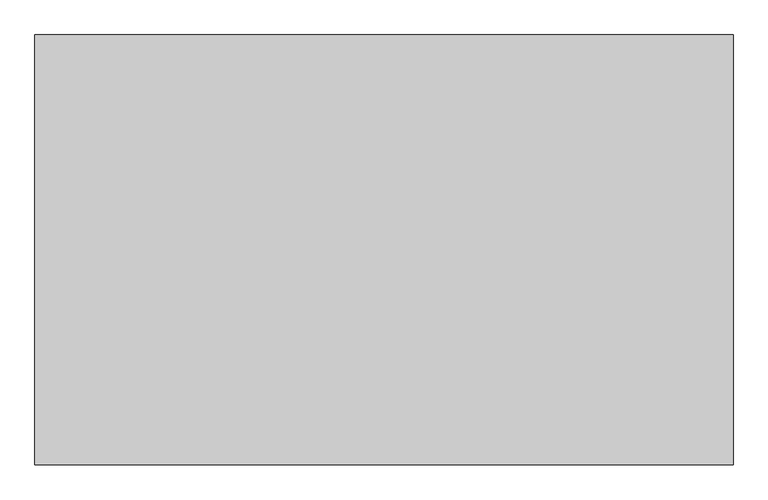
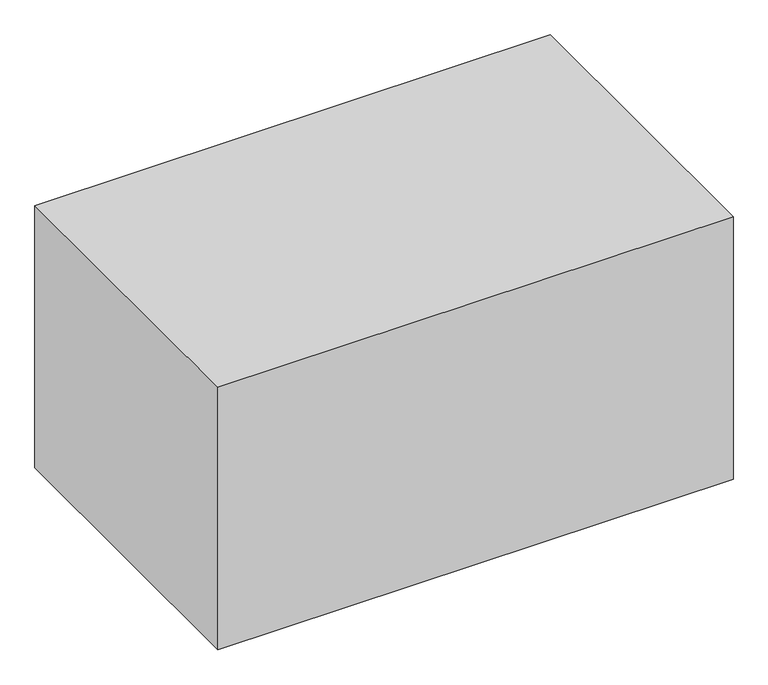
"""IFC4 building model written with IfcOpenShell, lengths in millimetres: proxy geometry, Space Planning Box_hec : Space Planning Box_hec."""

from ifc_helpers import new_model, si_unit, origin, origin_with_axes, place, context, project, spatial, polyline, outline, extrude, source, transform, mapped, element, save


def generic_models_8c4134a9(model_context):
    return source(origin(), model_context, "Body", "SweptSolid", [
        extrude(outline(polyline([(3250.0, 2000.0), (3250.0, -2000.0), (-3250.0, -2000.0), (-3250.0, 2000.0), (3250.0, 2000.0)])), origin_with_axes(), (0.0, 0.0, 1.0), 3500.0),
    ])


if __name__ == "__main__":
    model = new_model("IFC4")
    model_context = context("Model", 3, world=origin())
    ifc_project = project(units=[si_unit("LENGTHUNIT", "METRE", prefix="MILLI")], contexts=[model_context])
    site = spatial("IfcSite", under=ifc_project)
    building = spatial("IfcBuilding", under=site)
    placement = place(None, origin())
    generic_models_shape = generic_models_8c4134a9(model_context)
    element("IfcBuildingElementProxy", 1, Name="Space Planning Box_hec : Space Planning Box_hec", ObjectType="Space Planning Box_hec : Space Planning Box_hec", at=placement, inside=building, context=model_context, shape_type="MappedRepresentation", body=[
        mapped(generic_models_shape, transform((0.0, 0.0, 0.0), x_axis=(1.0, 0.0, 0.0), y_axis=(0.0, 1.0, 0.0), z_axis=(0.0, 0.0, 1.0))),
    ])
    save(model, "model.ifc")

# Revit data of these elements
# Type "Space Planning Box_hec : Space Planning Box_hec"
#   Type Comments = "..."
#   Room Name [instance default] = "?"
#   Interior Finish [instance default] = ""
#   Exterior Finish [instance default] = ""
#   Department [instance default] = ""
#   Assembly Code = "..."
#   ceiling height [instance default] = 0
#   Width [instance default] = 1524 mm
#   Program Area [instance default] = 0.00 m²
#   Length [instance default] = 1524 mm
#   Height [instance default] = 1524 mm
#   Area [instance default] = 2.32258 m²
#   Fill Color [instance default] = Cyan
#   Default Elevation = 0
# Element 1 (IfcBuildingElementProxy, "Space Planning Box_hec : Space Planning Box_hec")
#   Room Name = "Manager Office-1"
#   Exterior Finish = "RF1..N/A,,EW1..N/A..N/A"
#   Department = "AR"
#   Width = 6500 mm
#   Program Area = 26.00 m²
#   Length = 4000 mm
#   Height = 3500 mm
#   Area = 26.00 m²
#   Materials on its faces: "Cyan"
# Materials
#   "Cyan": class "Generic", colour RGB 0 255 255, transparency 0.2, Cost = 0
